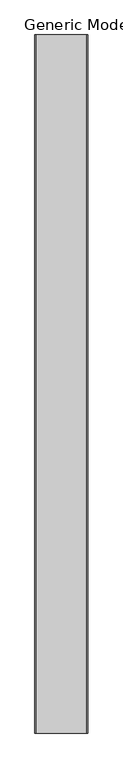
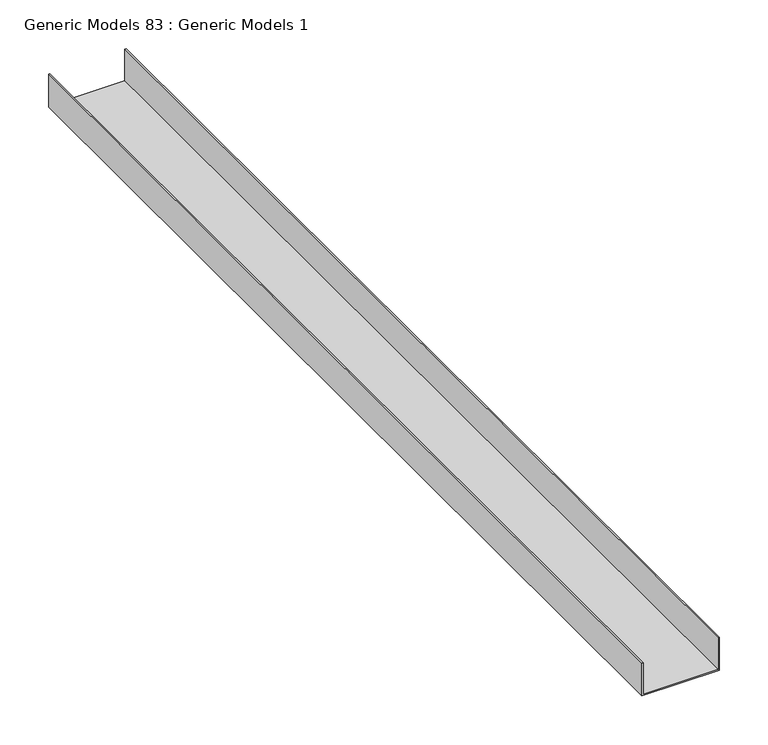
"""IFC4 building model written with IfcOpenShell, lengths in millimetres: proxy geometry, Generic Models 83 : Generic Models 1."""

import ifcopenshell
import ifcopenshell.guid

model = None  # the IFC model being written
_history = None  # IfcOwnerHistory: only IFC2X3 demands one
_inside = {}  # id of a spatial element -> (the spatial element, [elements in it])
_under = {}  # id of a project, library or spatial element -> (it, [spatial elements below it])
_declared = {}  # id of a project -> (the project, [libraries it declares])
_typed = {}  # id of a type object -> (the type object, [elements of that type])
_made_of = {}  # id of a material, layer set ... -> (it, [elements and type objects made of it])


def new_model(schema):
    """Start an empty IFC model of exactly this schema.

    Asked for "IFC4X3", IfcOpenShell would pick the latest addendum, in which some entities
    have other attributes; the version numbers below select the first issue.
    IFC2X3 requires an IfcOwnerHistory on every rooted entity: one is made here for all.
    """
    global model, _history
    if schema == "IFC4X3":
        model = ifcopenshell.file(schema_version=(4, 3, 0, 0))
    else:
        model = ifcopenshell.file(schema=schema)
    _inside.clear()
    _under.clear()
    _declared.clear()
    _typed.clear()
    _made_of.clear()
    _history = None
    if model.schema == "IFC2X3":
        org = make("IfcOrganization", Name="unknown")
        user = make(
            "IfcPersonAndOrganization",
            ThePerson=make("IfcPerson", FamilyName="unknown"),
            TheOrganization=org,
        )
        app = make(
            "IfcApplication",
            ApplicationDeveloper=org,
            Version="unknown",
            ApplicationFullName="unknown",
            ApplicationIdentifier="unknown",
        )
        _history = make(
            "IfcOwnerHistory",
            OwningUser=user,
            OwningApplication=app,
            ChangeAction="ADDED",
            CreationDate=0,
        )
    return model


def make(cls, **values):
    """One entity of the class cls with the attributes given. An attribute that is None is left unset."""
    return model.create_entity(
        cls, **{name: value for name, value in values.items() if value is not None}
    )


def rooted(cls, **values):
    """An entity with a GlobalId (a new one), such as an element, a storey or a relation."""
    return make(cls, GlobalId=ifcopenshell.guid.new(), OwnerHistory=_history, **values)


def si_unit(unit_type, name, prefix=None):
    """IfcSIUnit, for example si_unit("LENGTHUNIT", "METRE", prefix="MILLI")."""
    return make("IfcSIUnit", UnitType=unit_type, Prefix=prefix, Name=name)


def assignment(units):
    """IfcUnitAssignment: the units of a project."""
    return None if units is None else make("IfcUnitAssignment", Units=units)


def point(xyz):
    """IfcCartesianPoint."""
    return None if xyz is None else make("IfcCartesianPoint", Coordinates=xyz)


def direction(xyz):
    """IfcDirection."""
    return None if xyz is None else make("IfcDirection", DirectionRatios=xyz)


def frame(location, z_axis=None, x_axis=None):
    """IfcAxis2Placement3D, a coordinate frame: its origin and axes. An axis left out is left unset."""
    return make(
        "IfcAxis2Placement3D",
        Location=point(location),
        Axis=direction(z_axis),
        RefDirection=direction(x_axis),
    )


def origin():
    """The frame at (0, 0, 0) with its axes left unset."""
    return frame((0.0, 0.0, 0.0))


def place(relative_to, where):
    """IfcLocalPlacement: puts the frame where relative to a parent placement (None: the world)."""
    return make(
        "IfcLocalPlacement", PlacementRelTo=relative_to, RelativePlacement=where
    )


def context(
    kind, dimensions, precision=None, world=None, true_north=None, identifier=None
):
    """IfcGeometricRepresentationContext, for example the 3D "Model" context."""
    return make(
        "IfcGeometricRepresentationContext",
        ContextIdentifier=identifier,
        ContextType=kind,
        CoordinateSpaceDimension=dimensions,
        Precision=precision,
        WorldCoordinateSystem=world,
        TrueNorth=true_north,
    )


def project(units=None, contexts=None):
    """IfcProject with its units and contexts."""
    return rooted(
        "IfcProject",
        Name="project",
        RepresentationContexts=contexts,
        UnitsInContext=assignment(units),
    )


def spatial(cls, under=None, at=None, **own):
    """A site, building, storey or space (cls), placed at a placement, below another one or the project."""
    s = rooted(cls, ObjectPlacement=at, **own)
    if under is not None:
        _under.setdefault(under.id(), (under, []))[1].append(s)
    return s


def polyline(points):
    """IfcPolyline through the points."""
    return make("IfcPolyline", Points=[point(p) for p in points])


def outline(outer, holes=None, kind="AREA"):
    """IfcArbitraryClosedProfileDef: a profile drawn as a closed curve; with holes, ...WithVoids."""
    if holes is None:
        return make("IfcArbitraryClosedProfileDef", ProfileType=kind, OuterCurve=outer)
    return make(
        "IfcArbitraryProfileDefWithVoids",
        ProfileType=kind,
        OuterCurve=outer,
        InnerCurves=holes,
    )


def extrude(swept, where, along, depth):
    """IfcExtrudedAreaSolid: the profile swept, set in the frame where, extruded along a direction by depth."""
    return make(
        "IfcExtrudedAreaSolid",
        SweptArea=swept,
        Position=where,
        ExtrudedDirection=direction(along),
        Depth=depth,
    )


def shape(context_of_items, identifier, shape_type, items):
    """IfcShapeRepresentation: the items that make up one representation, for example the "Body"."""
    return make(
        "IfcShapeRepresentation",
        ContextOfItems=context_of_items,
        RepresentationIdentifier=identifier,
        RepresentationType=shape_type,
        Items=items,
    )


def source(mapping_origin, context_of_items, identifier, shape_type, items):
    """IfcRepresentationMap: a shape defined once, which mapped items show again and again."""
    return make(
        "IfcRepresentationMap",
        MappingOrigin=mapping_origin,
        MappedRepresentation=shape(context_of_items, identifier, shape_type, items),
    )


def transform(
    local_origin,
    x_axis=None,
    y_axis=None,
    z_axis=None,
    scale=None,
    scale2=None,
    scale3=None,
    uniform=True,
):
    """IfcCartesianTransformationOperator3D, or its non-uniform kind. x_axis, y_axis, z_axis: its Axis1, 2, 3."""
    if uniform:
        return make(
            "IfcCartesianTransformationOperator3D",
            Axis1=direction(x_axis),
            Axis2=direction(y_axis),
            LocalOrigin=point(local_origin),
            Scale=scale,
            Axis3=direction(z_axis),
        )
    return make(
        "IfcCartesianTransformationOperator3DnonUniform",
        Axis1=direction(x_axis),
        Axis2=direction(y_axis),
        LocalOrigin=point(local_origin),
        Scale=scale,
        Axis3=direction(z_axis),
        Scale2=scale2,
        Scale3=scale3,
    )


def mapped(mapping_source, mapping_target):
    """IfcMappedItem: shows the shape of a source again, moved by a transform."""
    return make(
        "IfcMappedItem", MappingSource=mapping_source, MappingTarget=mapping_target
    )


def made_of(thing, what):
    """Note that an element or type object is made of a material, layer set ...; save() writes the relation."""
    if what is not None:
        _made_of.setdefault(what.id(), (what, []))[1].append(thing)
    return thing


def element(
    cls,
    number,
    at=None,
    inside=None,
    cuts=None,
    type_object=None,
    material=None,
    context=None,
    identifier="Body",
    shape_type=None,
    held_by="IfcProductDefinitionShape",
    body=None,
    shapes=None,
    **own,
):
    """One element of the class cls, such as IfcWall. Its Tag is "e" and its number.

    at: its placement. inside: the storey or other place that contains it. cuts: it is an
    opening in that element (IfcRelVoidsElement). A single representation is given by context,
    identifier, shape_type and body (its items); several are given by shapes. held_by: the class
    of the entity that holds the representations. save() writes the other relations.
    """
    e = rooted(cls, Tag="e%d" % number, ObjectPlacement=at, **own)
    if body is not None:
        shapes = [shape(context, identifier, shape_type, body)]
    if shapes is not None:
        e.Representation = make(held_by, Representations=shapes)
    if inside is not None:
        _inside.setdefault(inside.id(), (inside, []))[1].append(e)
    if cuts is not None:
        rooted(
            "IfcRelVoidsElement", RelatingBuildingElement=cuts, RelatedOpeningElement=e
        )
    if type_object is not None:
        _typed.setdefault(type_object.id(), (type_object, []))[1].append(e)
    return made_of(e, material)


def aggregate(whole, parts):
    """IfcRelAggregates: a whole, such as a stair, and the parts it consists of."""
    return rooted("IfcRelAggregates", RelatingObject=whole, RelatedObjects=parts)


def save(model, path):
    """Write the relations noted so far, then the file.

    IfcRelAggregates (storeys below a building ...), IfcRelContainedInSpatialStructure (elements
    in a storey), IfcRelDefinesByType, IfcRelAssociatesMaterial and IfcRelDeclares: one each for
    every whole, place, type object, material and project.
    """
    for whole, parts in _under.values():
        aggregate(whole, parts)
    for where, things in _inside.values():
        rooted(
            "IfcRelContainedInSpatialStructure",
            RelatedElements=things,
            RelatingStructure=where,
        )
    for kind, things in _typed.values():
        rooted("IfcRelDefinesByType", RelatedObjects=things, RelatingType=kind)
    for what, things in _made_of.values():
        rooted("IfcRelAssociatesMaterial", RelatedObjects=things, RelatingMaterial=what)
    for by, libraries in _declared.values():
        rooted("IfcRelDeclares", RelatingContext=by, RelatedDefinitions=libraries)
    model.write(path)


def generic_models_83_generic_models_1_169b68fe(model_context):
    return source(origin(), model_context, "Body", "SweptSolid", [
        extrude(outline(polyline([(2067.2531297, 46935.8735531), (2108.5281297, 46935.8735531), (2108.5281297, 46934.2860531), (2068.8406297, 46934.2860531), (2068.8406297, 46845.3860531), (2108.5281297, 46845.3860531), (2108.5281297, 46843.7985531), (2067.2531297, 46843.7985531), (2067.2531297, 46935.8735531)])), frame((0.0, 0.0, 0.0), z_axis=(0.0, 1.0, 0.0), x_axis=(0.0, 0.0, 1.0)), (0.0, 0.0, 1.0), 1219.2),
    ])


if __name__ == "__main__":
    model = new_model("IFC4")
    model_context = context("Model", 3, world=origin())
    ifc_project = project(units=[si_unit("LENGTHUNIT", "METRE", prefix="MILLI")], contexts=[model_context])
    site = spatial("IfcSite", under=ifc_project)
    building = spatial("IfcBuilding", under=site)
    placement = place(None, origin())
    generic_models_83_generic_models_1_shape = generic_models_83_generic_models_1_169b68fe(model_context)
    element("IfcBuildingElementProxy", 1, Name="Generic Models 83 : Generic Models 1", ObjectType="Generic Models 83 : Generic Models 1", at=placement, inside=building, context=model_context, shape_type="MappedRepresentation", body=[
        mapped(generic_models_83_generic_models_1_shape, transform((0.0, 0.0, 0.0), x_axis=(1.0, 0.0, 0.0), y_axis=(0.0, 1.0, 0.0), z_axis=(0.0, 0.0, 1.0))),
    ])
    save(model, "model.ifc")

# Revit data of these elements
# Element 1 (IfcBuildingElementProxy, "Generic Models 83 : Generic Models 1")
#   Materials on its faces: "DEEP LEG OF DEFLECTION TRACK (2\" MIN. DEFLECTION)"
# Materials
#   "DEEP LEG OF DEFLECTION TRACK (2\" MIN. DEFLECTION)": class "Unassigned", colour RGB 210 209 208, transparency 0, Keynote = "M05121300.02", Cost = 0
